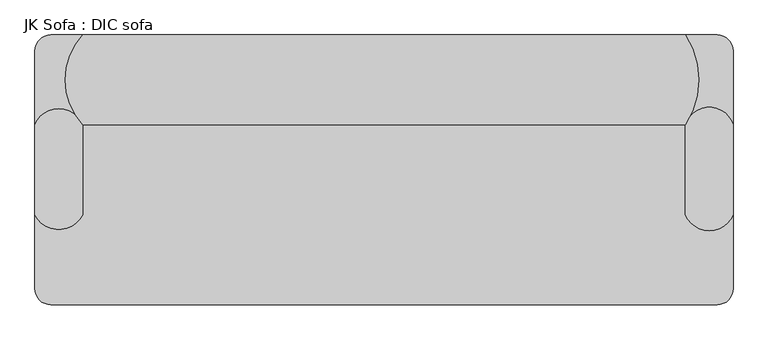
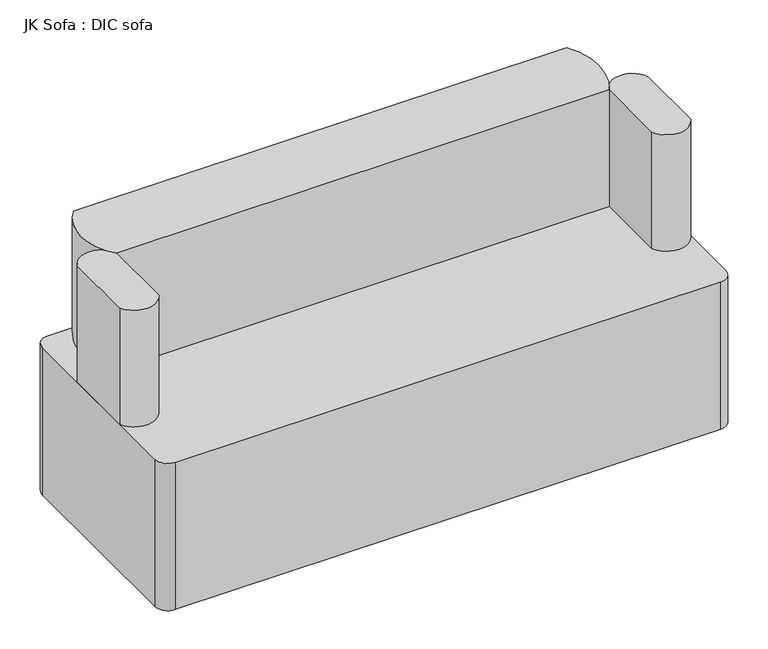
"""IFC4 building model written with IfcOpenShell, lengths in millimetres: furniture geometry, JK Sofa : DIC sofa."""

from ifc_helpers import new_model, si_unit, point, frame, frame_2d, origin, origin_with_axes, place, context, project, spatial, polyline, circle_curve, trimmed, segment, composite_curve, outline, extrude, source, transform, mapped, element, save


def jk_sofa_dic_sofa_e43bf39f(model_context):
    return source(origin(), model_context, "Body", "SweptSolid", [
        extrude(outline(composite_curve([segment(polyline([(903.2573665, 177.4788629), (-1027.1426335, 177.4788629)]), True, "CONTINUOUS"), segment(trimmed(circle_curve(frame_2d((-867.5613896, 321.4121962)), 214.9022518), [point((-1027.1426335, 177.4788629))], [point((-1027.1426335, 465.3455296))], False, "CARTESIAN"), True, "CONTINUOUS"), segment(polyline([(-1027.1426335, 465.3455296), (903.2573665, 465.3455296)]), True, "CONTINUOUS"), segment(trimmed(circle_curve(frame_2d((677.8181811, 321.4121962)), 267.4689342), [point((903.2573665, 465.3455296))], [point((903.2573665, 177.4788629))], False, "CARTESIAN"), True, "CONTINUOUS")], self_intersect=False)), frame((0.0, 0.0, 609.6), z_axis=(0.0, 0.0, 1.0), x_axis=(1.0, 0.0, 0.0)), (0.0, 0.0, 1.0), 482.6),
        extrude(outline(composite_curve([segment(polyline([(-1179.5426335, -110.3878038), (-1179.5426335, 177.4788629)]), True, "CONTINUOUS"), segment(trimmed(circle_curve(frame_2d((-1103.3426335, 147.712096)), 81.8077039), [point((-1179.5426335, 177.4788629))], [point((-1027.1426335, 177.4788629))], False, "CARTESIAN"), True, "CONTINUOUS"), segment(polyline([(-1027.1426335, 177.4788629), (-1027.1426335, -110.3878038)]), True, "CONTINUOUS"), segment(trimmed(circle_curve(frame_2d((-1103.3426335, -73.3296897)), 84.733369), [point((-1027.1426335, -110.3878038))], [point((-1179.5426335, -110.3878038))], False, "CARTESIAN"), True, "CONTINUOUS")], self_intersect=False)), frame((0.0, 0.0, 609.6), z_axis=(0.0, 0.0, 1.0), x_axis=(1.0, 0.0, 0.0)), (0.0, 0.0, 1.0), 482.6),
        extrude(outline(composite_curve([segment(polyline([(1055.6573665, 177.4788629), (1055.6573665, -110.3878038)]), True, "CONTINUOUS"), segment(trimmed(circle_curve(frame_2d((979.4573665, -78.2408831)), 82.7034734), [point((1055.6573665, -110.3878038))], [point((903.2573665, -110.3878038))], False, "CARTESIAN"), True, "CONTINUOUS"), segment(polyline([(903.2573665, -110.3878038), (903.2573665, 177.4788629)]), True, "CONTINUOUS"), segment(trimmed(circle_curve(frame_2d((979.4573665, 153.7481356)), 79.809695), [point((903.2573665, 177.4788629))], [point((1055.6573665, 177.4788629))], False, "CARTESIAN"), True, "CONTINUOUS")], self_intersect=False)), frame((0.0, 0.0, 609.6), z_axis=(0.0, 0.0, 1.0), x_axis=(1.0, 0.0, 0.0)), (0.0, 0.0, 1.0), 482.6),
        extrude(outline(composite_curve([segment(trimmed(circle_curve(frame_2d((1004.8573665, 414.5455296)), 50.8), [point((1004.8573665, 465.3455296))], [point((1055.6573665, 414.5455296))], False, "CARTESIAN"), True, "CONTINUOUS"), segment(polyline([(1055.6573665, 414.5455296), (1055.6573665, -347.4544704)]), True, "CONTINUOUS"), segment(trimmed(circle_curve(frame_2d((1004.8573665, -347.4544704)), 50.8), [point((1055.6573665, -347.4544704))], [point((1004.8573665, -398.2544704))], False, "CARTESIAN"), True, "CONTINUOUS"), segment(polyline([(1004.8573665, -398.2544704), (-1128.7426335, -398.2544704)]), True, "CONTINUOUS"), segment(trimmed(circle_curve(frame_2d((-1128.7426335, -347.4544704)), 50.8), [point((-1128.7426335, -398.2544704))], [point((-1179.5426335, -347.4544704))], False, "CARTESIAN"), True, "CONTINUOUS"), segment(polyline([(-1179.5426335, -347.4544704), (-1179.5426335, 414.5455296)]), True, "CONTINUOUS"), segment(trimmed(circle_curve(frame_2d((-1128.7426335, 414.5455296)), 50.8), [point((-1179.5426335, 414.5455296))], [point((-1128.7426335, 465.3455296))], False, "CARTESIAN"), True, "CONTINUOUS"), segment(polyline([(-1128.7426335, 465.3455296), (1004.8573665, 465.3455296)]), True, "CONTINUOUS")], self_intersect=False)), origin_with_axes(), (0.0, 0.0, 1.0), 609.6),
    ])


if __name__ == "__main__":
    model = new_model("IFC4")
    model_context = context("Model", 3, world=origin())
    ifc_project = project(units=[si_unit("LENGTHUNIT", "METRE", prefix="MILLI")], contexts=[model_context])
    site = spatial("IfcSite", under=ifc_project)
    building = spatial("IfcBuilding", under=site)
    placement = place(None, origin())
    jk_sofa_dic_sofa_shape = jk_sofa_dic_sofa_e43bf39f(model_context)
    element("IfcFurniture", 1, ObjectType="JK Sofa : DIC sofa", at=placement, inside=building, context=model_context, shape_type="MappedRepresentation", body=[
        mapped(jk_sofa_dic_sofa_shape, transform((0.0, 0.0, 0.0), x_axis=(1.0, 0.0, 0.0), y_axis=(0.0, 1.0, 0.0), z_axis=(0.0, 0.0, 1.0))),
    ])
    save(model, "model.ifc")

# Revit data of these elements
# Type "JK Sofa : DIC sofa"
#   Width = 7' - 4"
#   Seat Height = 2' - 0"
#   Depth = 2' - 10"
#   Corner Radius = 0' - 2"
#   Back Height = 3' - 7"
#   Arm Width = 0' - 6"
#   Status [instance default] = none
#   Default Elevation = 0
